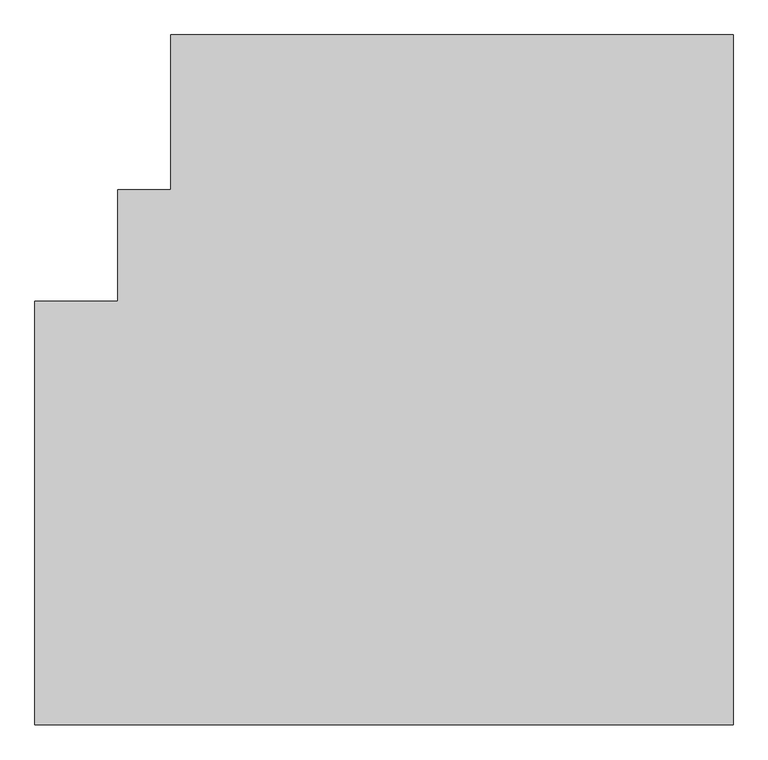
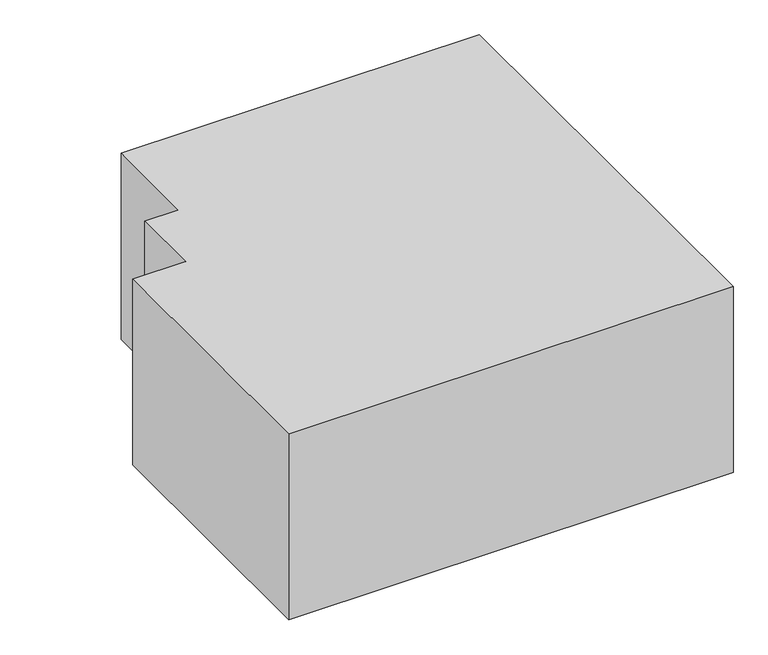
"""IFC4 building model written with IfcOpenShell, lengths in millimetres: proxy geometry, 0_3d_modell."""

from ifc_helpers import new_model, si_unit, origin, origin_with_axes, place, context, project, spatial, polyline, outline, extrude, source, transform, mapped, element, save


def generic_models_472136ed(model_context):
    return source(origin(), model_context, "Body", "SweptSolid", [
        extrude(outline(polyline([(5650.159292, 5582.8619019), (5650.159292, 0.0), (0.0, 0.0), (0.159292, 3427.8619019), (670.159292, 3427.8619019), (670.159292, 4327.8619019), (1100.159292, 4327.8619019), (1100.159292, 5582.8619019), (5650.159292, 5582.8619019)])), origin_with_axes(), (0.0, 0.0, 1.0), 2500.0),
    ])


if __name__ == "__main__":
    model = new_model("IFC4")
    model_context = context("Model", 3, world=origin())
    ifc_project = project(units=[si_unit("LENGTHUNIT", "METRE", prefix="MILLI")], contexts=[model_context])
    site = spatial("IfcSite", under=ifc_project)
    building = spatial("IfcBuilding", under=site)
    placement = place(None, origin())
    generic_models_shape = generic_models_472136ed(model_context)
    element("IfcBuildingElementProxy", 1, Name="0_3d_modell", ObjectType="0_3d_modell", at=placement, inside=building, context=model_context, shape_type="MappedRepresentation", body=[
        mapped(generic_models_shape, transform((0.0, 0.0, 0.0), x_axis=(1.0, 0.0, 0.0), y_axis=(0.0, 1.0, 0.0), z_axis=(0.0, 0.0, 1.0))),
    ])
    save(model, "model.ifc")

# Revit data of these elements
# Element 1 (IfcBuildingElementProxy, "0_3d_modell")
#   Materials on its faces: "*1"
# Materials
#   "*1": class "Unassigned", colour RGB 175 175 175, transparency 0
